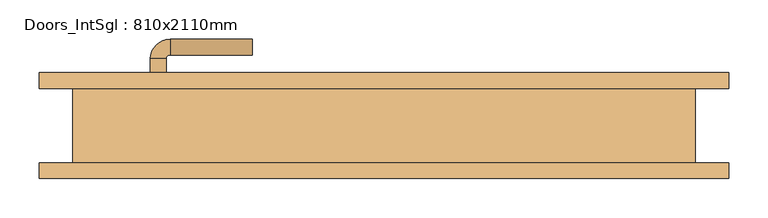
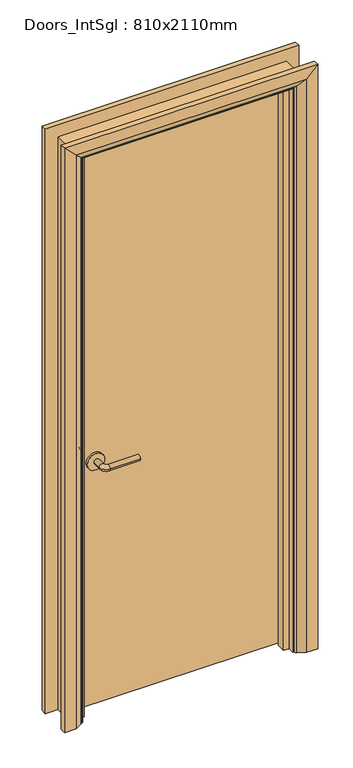
"""IFC4 building model written with IfcOpenShell, lengths in millimetres: door geometry, Doors_IntSgl : 810x2110mm."""

from ifc_helpers import new_model, si_unit, point, frame, frame_2d, origin, place, context, project, spatial, polyline, circle_curve, ellipse_curve, trimmed, segment, composite_curve, outline, extrude, faceted_brep, source, transform, mapped, element, save
from ifc_brep_helpers import plane_surface, cylinder_surface, revolved_surface, advanced_brep


def doors_intsgl_810x2110mm_acea5367(model_context):
    return source(origin(), model_context, "Body", "SolidModel", [
        advanced_brep(
        [(-298.0, 1.5, 900.0), (-278.0, 1.5, 900.0), (-278.0, -28.5, 900.0), (-298.0, -28.5, 900.0), (-273.0, -33.5, 900.0), (-273.0, -53.5, 900.0), (-168.0, -53.5, 900.0), (-168.0, -33.5, 900.0)],
        [
            (0, 1, circle_curve(frame((-288.0, 1.5, 900.0), z_axis=(0.0, 1.0, 0.0), x_axis=(1.0, 0.0, 0.0)), 10.0)),
            (1, 0, circle_curve(frame((-288.0, 1.5, 900.0), z_axis=(0.0, 1.0, 0.0), x_axis=(1.0, 0.0, 0.0)), 10.0)),
            (1, 2),
            (2, 3, circle_curve(frame((-288.0, -28.5, 900.0), z_axis=(0.0, 1.0, 0.0), x_axis=(1.0, 0.0, 0.0)), 10.0)),
            (3, 0),
            (3, 2, circle_curve(frame((-288.0, -28.5, 900.0), z_axis=(0.0, 1.0, 0.0), x_axis=(1.0, 0.0, 0.0)), 10.0)),
            (4, 5, circle_curve(frame((-273.0, -43.5, 900.0), z_axis=(-1.0, 0.0, 0.0), x_axis=(0.0, 1.0, 0.0)), 10.0)),
            (5, 3, circle_curve(frame((-273.0, -28.5, 900.0), z_axis=(0.0, 0.0, -1.0), x_axis=(-1.0, 0.0, 0.0)), 25.0)),
            (2, 4, circle_curve(frame((-273.0, -28.5, 900.0), z_axis=(0.0, 0.0, 1.0), x_axis=(-1.0, 0.0, 0.0)), 5.0)),
            (5, 4, circle_curve(frame((-273.0, -43.5, 900.0), z_axis=(-1.0, 0.0, 0.0), x_axis=(0.0, 1.0, 0.0)), 10.0)),
            (6, 7, circle_curve(frame((-168.0, -43.5, 900.0), z_axis=(1.0, 0.0, 0.0), x_axis=(0.0, 1.0, 0.0)), 10.0)),
            (7, 6, circle_curve(frame((-168.0, -43.5, 900.0), z_axis=(1.0, 0.0, 0.0), x_axis=(0.0, 1.0, 0.0)), 10.0)),
            (4, 7),
            (6, 5),
        ],
        [
            plane_surface(frame((-288.0, 1.5, 900.0), z_axis=(0.0, 1.0, 0.0), x_axis=(0.0, 0.0, 1.0))),
            cylinder_surface(frame((-288.0, 1.5, 900.0), z_axis=(0.0, 1.0, 0.0), x_axis=(1.0, 0.0, 0.0)), 10.0),
            revolved_surface(trimmed(ellipse_curve(frame((-288.0, -28.5, 900.0), z_axis=(0.0, -1.0, 0.0), x_axis=(1.0, 0.0, 0.0)), 10.0, 10.0), [point((-298.0, -28.5, 900.0))], [point((-278.0, -28.5, 900.0))], True, "CARTESIAN"), (-273.0, -28.5, 900.0), (0.0, 0.0, -1.0)),
            revolved_surface(trimmed(ellipse_curve(frame((-288.0, -28.5, 900.0), z_axis=(0.0, -1.0, 0.0), x_axis=(1.0, 0.0, 0.0)), 10.0, 10.0), [point((-278.0, -28.5, 900.0))], [point((-298.0, -28.5, 900.0))], True, "CARTESIAN"), (-273.0, -28.5, 900.0), (0.0, 0.0, -1.0)),
            plane_surface(frame((-168.0, -43.5, 900.0), z_axis=(1.0, 0.0, 0.0), x_axis=(0.0, 0.0, 1.0))),
            cylinder_surface(frame((-273.0, -43.5, 900.0), z_axis=(-1.0, 0.0, 0.0), x_axis=(0.0, 1.0, 0.0)), 10.0),
        ],
        [
            (0, [[1, 2]]),
            (1, [[3, 4, 5, -2]]),
            (1, [[-5, 6, -3, -1]]),
            (2, [[7, 8, -4, 9]]),
            (3, [[10, -9, -6, -8]]),
            (4, [[11, 12]]),
            (5, [[13, -11, 14, -7]]),
            (5, [[-14, -12, -13, -10]]),
        ],
    ),
        extrude(outline(composite_curve([segment(trimmed(circle_curve(frame_2d((900.0, -290.5)), 30.0), [point((900.0, -320.5))], [point((900.0, -260.5))], False, "CARTESIAN"), True, "CONTINUOUS"), segment(trimmed(circle_curve(frame_2d((900.0, -290.5)), 30.0), [point((900.0, -260.5))], [point((900.0, -320.5))], False, "CARTESIAN"), True, "CONTINUOUS")], self_intersect=False)), frame((0.0, 1.5, 0.0), z_axis=(0.0, 1.0, 0.0), x_axis=(0.0, 0.0, 1.0)), (0.0, 0.0, 1.0), 8.0),
        advanced_brep(
        [(-298.0, 55.5, 900.0), (-278.0, 55.5, 900.0), (-298.0, 85.5, 900.0), (-278.0, 85.5, 900.0), (-273.0, 90.5, 900.0), (-273.0, 110.5, 900.0), (-168.0, 110.5, 900.0), (-168.0, 90.5, 900.0)],
        [
            (0, 1, circle_curve(frame((-288.0, 55.5, 900.0), z_axis=(0.0, -1.0, 0.0), x_axis=(1.0, 0.0, 0.0)), 10.0)),
            (1, 0, circle_curve(frame((-288.0, 55.5, 900.0), z_axis=(0.0, -1.0, 0.0), x_axis=(1.0, 0.0, 0.0)), 10.0)),
            (0, 2),
            (2, 3, circle_curve(frame((-288.0, 85.5, 900.0), z_axis=(0.0, -1.0, 0.0), x_axis=(1.0, 0.0, 0.0)), 10.0)),
            (3, 1),
            (3, 2, circle_curve(frame((-288.0, 85.5, 900.0), z_axis=(0.0, -1.0, 0.0), x_axis=(1.0, 0.0, 0.0)), 10.0)),
            (4, 3, circle_curve(frame((-273.0, 85.5, 900.0), z_axis=(0.0, 0.0, 1.0), x_axis=(-1.0, 0.0, 0.0)), 5.0)),
            (2, 5, circle_curve(frame((-273.0, 85.5, 900.0), z_axis=(0.0, 0.0, -1.0), x_axis=(-1.0, 0.0, 0.0)), 25.0)),
            (5, 4, circle_curve(frame((-273.0, 100.5, 900.0), z_axis=(-1.0, 0.0, 0.0), x_axis=(0.0, -1.0, 0.0)), 10.0)),
            (4, 5, circle_curve(frame((-273.0, 100.5, 900.0), z_axis=(-1.0, 0.0, 0.0), x_axis=(0.0, -1.0, 0.0)), 10.0)),
            (6, 7, circle_curve(frame((-168.0, 100.5, 900.0), z_axis=(1.0, 0.0, 0.0), x_axis=(0.0, -1.0, 0.0)), 10.0)),
            (7, 6, circle_curve(frame((-168.0, 100.5, 900.0), z_axis=(1.0, 0.0, 0.0), x_axis=(0.0, -1.0, 0.0)), 10.0)),
            (5, 6),
            (7, 4),
        ],
        [
            plane_surface(frame((-288.0, 55.5, 900.0), z_axis=(0.0, -1.0, 0.0), x_axis=(0.0, 0.0, 1.0))),
            cylinder_surface(frame((-288.0, 55.5, 900.0), z_axis=(0.0, -1.0, 0.0), x_axis=(1.0, 0.0, 0.0)), 10.0),
            revolved_surface(trimmed(ellipse_curve(frame((-288.0, 85.5, 900.0), z_axis=(0.0, -1.0, 0.0), x_axis=(1.0, 0.0, 0.0)), 10.0, 10.0), [point((-298.0, 85.5, 900.0))], [point((-278.0, 85.5, 900.0))], True, "CARTESIAN"), (-273.0, 85.5, 900.0), (0.0, 0.0, -1.0)),
            revolved_surface(trimmed(ellipse_curve(frame((-288.0, 85.5, 900.0), z_axis=(0.0, -1.0, 0.0), x_axis=(1.0, 0.0, 0.0)), 10.0, 10.0), [point((-278.0, 85.5, 900.0))], [point((-298.0, 85.5, 900.0))], True, "CARTESIAN"), (-273.0, 85.5, 900.0), (0.0, 0.0, -1.0)),
            plane_surface(frame((-168.0, 100.5, 900.0), z_axis=(1.0, 0.0, 0.0), x_axis=(0.0, 0.0, 1.0))),
            cylinder_surface(frame((-273.0, 100.5, 900.0), z_axis=(-1.0, 0.0, 0.0), x_axis=(0.0, -1.0, 0.0)), 10.0),
        ],
        [
            (0, [[1, 2]]),
            (1, [[-1, 3, 4, 5]]),
            (1, [[-2, -5, 6, -3]]),
            (2, [[7, -4, 8, 9]]),
            (3, [[-8, -6, -7, 10]]),
            (4, [[11, 12]]),
            (5, [[-9, 13, -12, 14]]),
            (5, [[-10, -14, -11, -13]]),
        ],
    ),
        extrude(outline(composite_curve([segment(trimmed(circle_curve(frame_2d((900.0, -290.5)), 30.0), [point((900.0, -320.5))], [point((900.0, -260.5))], False, "CARTESIAN"), True, "CONTINUOUS"), segment(trimmed(circle_curve(frame_2d((900.0, -290.5)), 30.0), [point((900.0, -260.5))], [point((900.0, -320.5))], False, "CARTESIAN"), True, "CONTINUOUS")], self_intersect=False)), frame((0.0, 47.5, 0.0), z_axis=(0.0, 1.0, 0.0), x_axis=(0.0, 0.0, 1.0)), (0.0, 0.0, 1.0), 8.0),
        extrude(outline(polyline([(363.0, 9.5), (-363.0, 9.5), (-363.0, 47.5), (363.0, 47.5), (363.0, 9.5)])), frame((0.0, 0.0, 8.0), z_axis=(0.0, 0.0, 1.0), x_axis=(1.0, 0.0, 0.0)), (0.0, 0.0, 1.0), 2060.0),
        advanced_brep(
        [(440.0, 67.5, 0.0), (440.0, 47.5, 0.0), (370.0, 47.5, 0.0), (374.0, 53.5, 0.0), (400.0, 67.5, 0.0), (440.0, 67.5, 2145.0), (440.0, 47.5, 2145.0), (-440.0, 47.5, 2145.0), (-440.0, 47.5, 0.0), (-370.0, 47.5, 0.0), (-370.0, 47.5, 2075.0), (370.0, 47.5, 2075.0), (374.0, 53.5, 2079.0), (400.0, 67.5, 2105.0), (-400.0, 67.5, 2105.0), (-400.0, 67.5, 0.0), (-440.0, 67.5, 0.0), (-440.0, 67.5, 2145.0), (-374.0, 53.5, 2079.0), (-374.0, 53.5, 0.0)],
        [
            (0, 1),
            (1, 2),
            (2, 3, circle_curve(frame((378.0, 46.5, 0.0), z_axis=(0.0, 0.0, -1.0), x_axis=(1.0, 0.0, 0.0)), 8.0622577)),
            (3, 4),
            (4, 0),
            (0, 5),
            (5, 6),
            (6, 1),
            (6, 7),
            (7, 8),
            (8, 9),
            (9, 10),
            (10, 11),
            (11, 2),
            (11, 12, ellipse_curve(frame((378.0, 46.5, 2083.0), z_axis=(0.7071067811865475, 0.0, -0.7071067811865475), x_axis=(-0.7071067811865474, 0.0, -0.7071067811865476)), 11.4017543, 8.0622577)),
            (12, 3),
            (12, 13),
            (13, 4),
            (13, 14),
            (14, 15),
            (15, 16),
            (16, 17),
            (17, 5),
            (17, 7),
            (10, 18, ellipse_curve(frame((-378.0, 46.5, 2083.0), z_axis=(0.7071067811865475, 0.0, 0.7071067811865475), x_axis=(0.7071067811865476, 0.0, -0.7071067811865474)), 11.4017543, 8.0622577)),
            (18, 12),
            (18, 14),
            (15, 19),
            (19, 9, circle_curve(frame((-378.0, 46.5, 0.0), z_axis=(0.0, 0.0, -1.0), x_axis=(-1.0, 0.0, 0.0)), 8.0622577)),
            (8, 16),
            (19, 18),
        ],
        [
            plane_surface(frame((370.0, 47.5, 0.0), z_axis=(0.0, 0.0, -1.0), x_axis=(0.0, -1.0, 0.0))),
            plane_surface(frame((440.0, 67.5, 0.0), z_axis=(1.0, 0.0, 0.0), x_axis=(0.0, 0.0, 1.0))),
            plane_surface(frame((440.0, 47.5, 0.0), z_axis=(0.0, -1.0, 0.0), x_axis=(0.0, 0.0, 1.0))),
            cylinder_surface(frame((378.0, 46.5, 0.0), z_axis=(0.0, 0.0, -1.0), x_axis=(1.0, 0.0, 0.0)), 8.0622577),
            plane_surface(frame((374.0, 53.5, 0.0), z_axis=(-0.4740998230350126, 0.880471099922178, 0.0), x_axis=(0.0, 0.0, 1.0))),
            plane_surface(frame((400.0, 67.5, 0.0), z_axis=(0.0, 1.0, 0.0), x_axis=(0.0, 0.0, 1.0))),
            plane_surface(frame((440.0, 67.5, 2145.0), z_axis=(0.0, 0.0, 1.0), x_axis=(-1.0, 0.0, 0.0))),
            cylinder_surface(frame((370.0, 46.5, 2083.0), z_axis=(1.0, 0.0, 0.0), x_axis=(0.0, 0.0, 1.0)), 8.0622577),
            plane_surface(frame((374.0, 53.5, 2079.0), z_axis=(0.0, 0.8804710999221764, -0.4740998230350154), x_axis=(-1.0, 0.0, 0.0))),
            plane_surface(frame((-370.0, 47.5, 0.0), z_axis=(0.0, 0.0, -1.0), x_axis=(0.0, -1.0, 0.0))),
            plane_surface(frame((-440.0, 67.5, 2145.0), z_axis=(-1.0, 0.0, 0.0), x_axis=(0.0, 0.0, -1.0))),
            cylinder_surface(frame((-378.0, 46.5, 2075.0), z_axis=(0.0, 0.0, 1.0), x_axis=(-1.0, 0.0, 0.0)), 8.0622577),
            plane_surface(frame((-374.0, 53.5, 2079.0), z_axis=(0.47409982303501824, 0.8804710999221749, 0.0), x_axis=(0.0, 0.0, -1.0))),
        ],
        [
            (0, [[1, 2, 3, 4, 5]]),
            (1, [[-1, 6, 7, 8]]),
            (2, [[-2, -8, 9, 10, 11, 12, 13, 14]]),
            (3, [[-3, -14, 15, 16]]),
            (4, [[-4, -16, 17, 18]]),
            (5, [[-5, -18, 19, 20, 21, 22, 23, -6]]),
            (6, [[-7, -23, 24, -9]]),
            (7, [[-15, -13, 25, 26]]),
            (8, [[-17, -26, 27, -19]]),
            (9, [[-21, 28, 29, -11, 30]]),
            (10, [[-24, -22, -30, -10]]),
            (11, [[-25, -12, -29, 31]]),
            (12, [[-27, -31, -28, -20]]),
        ],
    ),
        extrude(outline(polyline([(0.0, -365.0), (0.0, -346.0), (2051.0, -346.0), (2051.0, 346.0), (0.0, 346.0), (0.0, 365.0), (2070.0, 365.0), (2070.0, -365.0), (0.0, -365.0)])), frame((0.0, -24.5, 0.0), z_axis=(0.0, 1.0, 0.0), x_axis=(0.0, 0.0, 1.0)), (0.0, 0.0, 1.0), 32.0),
        advanced_brep(
        [(-440.0, -67.5, 0.0), (-440.0, -47.5, 0.0), (-370.0, -47.5, 0.0), (-374.0, -53.5, 0.0), (-400.0, -67.5, 0.0), (-440.0, -67.5, 2145.0), (-440.0, -47.5, 2145.0), (-370.0, -47.5, 2075.0), (-374.0, -53.5, 2079.0), (-400.0, -67.5, 2105.0), (440.0, -67.5, 2145.0), (440.0, -47.5, 2145.0), (370.0, -47.5, 2075.0), (374.0, -53.5, 2079.0), (400.0, -67.5, 2105.0), (440.0, -67.5, 0.0), (400.0, -67.5, 0.0), (374.0, -53.5, 0.0), (370.0, -47.5, 0.0), (440.0, -47.5, 0.0)],
        [
            (0, 1),
            (1, 2),
            (2, 3, circle_curve(frame((-378.0, -46.5, 0.0), z_axis=(0.0, 0.0, -1.0), x_axis=(-1.0, 0.0, 0.0)), 8.0622577)),
            (3, 4),
            (4, 0),
            (0, 5),
            (5, 6),
            (6, 1),
            (6, 7),
            (7, 2),
            (7, 8, ellipse_curve(frame((-378.0, -46.5, 2083.0), z_axis=(-0.7071067811865475, 0.0, -0.7071067811865475), x_axis=(0.7071067811865474, 0.0, -0.7071067811865476)), 11.4017543, 8.0622577)),
            (8, 3),
            (8, 9),
            (9, 4),
            (9, 5),
            (5, 10),
            (10, 11),
            (11, 6),
            (11, 12),
            (12, 7),
            (12, 13, ellipse_curve(frame((378.0, -46.5, 2083.0), z_axis=(-0.7071067811865475, 0.0, 0.7071067811865475), x_axis=(-0.7071067811865476, 0.0, -0.7071067811865474)), 11.4017543, 8.0622577)),
            (13, 8),
            (13, 14),
            (14, 9),
            (14, 10),
            (15, 16),
            (16, 17),
            (17, 18, circle_curve(frame((378.0, -46.5, 0.0), z_axis=(0.0, 0.0, -1.0), x_axis=(1.0, 0.0, 0.0)), 8.0622577)),
            (18, 19),
            (19, 15),
            (10, 15),
            (19, 11),
            (18, 12),
            (17, 13),
            (16, 14),
        ],
        [
            plane_surface(frame((-370.0, -120.3010989, 0.0), z_axis=(0.0, 0.0, -1.0), x_axis=(1.0, 0.0, 0.0))),
            plane_surface(frame((-440.0, -67.5, 0.0), z_axis=(-1.0, 0.0, 0.0), x_axis=(0.0, 0.0, 1.0))),
            plane_surface(frame((-440.0, -47.5, 0.0), z_axis=(0.0, 1.0, 0.0), x_axis=(0.0, 0.0, 1.0))),
            cylinder_surface(frame((-378.0, -46.5, 0.0), z_axis=(0.0, 0.0, -1.0), x_axis=(-1.0, 0.0, 0.0)), 8.0622577),
            plane_surface(frame((-374.0, -53.5, 0.0), z_axis=(0.4740998230350183, -0.8804710999221749, 0.0), x_axis=(0.0, 0.0, 1.0))),
            plane_surface(frame((-400.0, -67.5, 0.0), z_axis=(0.0, -1.0, 0.0), x_axis=(0.0, 0.0, 1.0))),
            plane_surface(frame((-440.0, -67.5, 2145.0), z_axis=(0.0, 0.0, 1.0), x_axis=(1.0, 0.0, 0.0))),
            plane_surface(frame((-440.0, -47.5, 2145.0), z_axis=(0.0, 1.0, 0.0), x_axis=(1.0, 0.0, 0.0))),
            cylinder_surface(frame((-370.0, -46.5, 2083.0), z_axis=(-1.0, 0.0, 0.0), x_axis=(0.0, 0.0, 1.0)), 8.0622577),
            plane_surface(frame((-374.0, -53.5, 2079.0), z_axis=(0.0, -0.8804710999221749, -0.4740998230350183), x_axis=(1.0, 0.0, 0.0))),
            plane_surface(frame((-400.0, -67.5, 2105.0), z_axis=(0.0, -1.0, 0.0), x_axis=(1.0, 0.0, 0.0))),
            plane_surface(frame((370.0, -120.3010989, 0.0), z_axis=(0.0, 0.0, -1.0), x_axis=(-1.0, 0.0, 0.0))),
            plane_surface(frame((440.0, -67.5, 2145.0), z_axis=(1.0, 0.0, 0.0), x_axis=(0.0, 0.0, -1.0))),
            plane_surface(frame((440.0, -47.5, 2145.0), z_axis=(0.0, 1.0, 0.0), x_axis=(0.0, 0.0, -1.0))),
            cylinder_surface(frame((378.0, -46.5, 2075.0), z_axis=(0.0, 0.0, 1.0), x_axis=(1.0, 0.0, 0.0)), 8.0622577),
            plane_surface(frame((374.0, -53.5, 2079.0), z_axis=(-0.4740998230350183, -0.8804710999221749, 0.0), x_axis=(0.0, 0.0, -1.0))),
            plane_surface(frame((400.0, -67.5, 2105.0), z_axis=(0.0, -1.0, 0.0), x_axis=(0.0, 0.0, -1.0))),
        ],
        [
            (0, [[1, 2, 3, 4, 5]]),
            (1, [[-1, 6, 7, 8]]),
            (2, [[-2, -8, 9, 10]]),
            (3, [[-3, -10, 11, 12]]),
            (4, [[-4, -12, 13, 14]]),
            (5, [[-5, -14, 15, -6]]),
            (6, [[-7, 16, 17, 18]]),
            (7, [[-9, -18, 19, 20]]),
            (8, [[-11, -20, 21, 22]]),
            (9, [[-13, -22, 23, 24]]),
            (10, [[-15, -24, 25, -16]]),
            (11, [[26, 27, 28, 29, 30]]),
            (12, [[-17, 31, -30, 32]]),
            (13, [[-19, -32, -29, 33]]),
            (14, [[-21, -33, -28, 34]]),
            (15, [[-23, -34, -27, 35]]),
            (16, [[-25, -35, -26, -31]]),
        ],
    ),
        faceted_brep([(-365.0, 47.5, 0.0), (-365.0, -47.5, 0.0), (-397.0, -47.5, 0.0), (-397.0, 47.5, 0.0), (-365.0, 47.5, 2070.0), (-365.0, -47.5, 2070.0), (-397.0, -47.5, 2102.0), (-397.0, 47.5, 2102.0), (365.0, 47.5, 2070.0), (365.0, -47.5, 2070.0), (397.0, -47.5, 2102.0), (397.0, 47.5, 2102.0), (365.0, 47.5, 0.0), (397.0, 47.5, 0.0), (397.0, -47.5, 0.0), (365.0, -47.5, 0.0)], [[[0, 1, 2, 3]], [[1, 0, 4, 5]], [[2, 1, 5, 6]], [[3, 2, 6, 7]], [[0, 3, 7, 4]], [[5, 4, 8, 9]], [[6, 5, 9, 10]], [[7, 6, 10, 11]], [[4, 7, 11, 8]], [[12, 13, 14, 15]], [[9, 8, 12, 15]], [[10, 9, 15, 14]], [[11, 10, 14, 13]], [[8, 11, 13, 12]]]),
    ])


if __name__ == "__main__":
    model = new_model("IFC4")
    model_context = context("Model", 3, world=origin())
    ifc_project = project(units=[si_unit("LENGTHUNIT", "METRE", prefix="MILLI")], contexts=[model_context])
    site = spatial("IfcSite", under=ifc_project)
    building = spatial("IfcBuilding", under=site)
    placement = place(None, origin())
    doors_intsgl_810x2110mm_shape = doors_intsgl_810x2110mm_acea5367(model_context)
    element("IfcDoor", 1, ObjectType="Doors_IntSgl : 810x2110mm", at=placement, inside=building, context=model_context, shape_type="MappedRepresentation", body=[
        mapped(doors_intsgl_810x2110mm_shape, transform((0.0, 0.0, 0.0), x_axis=(1.0, 0.0, 0.0), y_axis=(0.0, 1.0, 0.0), z_axis=(0.0, 0.0, 1.0))),
    ])
    save(model, "model.ifc")

# Revit data of these elements
# Type "Doors_IntSgl : 810x2110mm"
#   Construction Type Id = "MDOOR"
#   Type Mark = "42"
#   Type Comments = "Internal Single"
#   Operation = "SingleSwingRight"
#   Manufacturer = "Revit"
#   Keynote = "L20"
#   Description = "Internal Single Door"
#   Analytic Construction = "Metal"
#   UnderCut = 8 mm
#   Tolerance = 2 mm
#   Thickness = 38 mm
#   Thermal Resistance (R) = 0.270117 (m²·K)/W
#   Structural Tolerance = 8 mm
#   StopDepth = 32 mm
#   Stop Thickness = 19 mm
#   Rough Width = 810 mm
#   Rough Height = 2110 mm
#   Height to Top Lock Rail = 1000 mm
#   Heat Transfer Coefficient (U) = 3.7021 W/(m²·K)
#   Handle Z Distance = 900 mm
#   Handle X Distance = 75 mm
#   Frame Thickness = 32 mm
#   Door Panel Width = 726 mm
#   Door Panel Thickness = 38 mm
#   Door Panel Offset = 0 mm
#   Height = 2110 mm
#   Width = 810 mm
#   Door Panel Height = 2060 mm
#   Architrave Setback = 5 mm
#   Vis - Ironmongery = yes
#   Material Ironmongery = Door - Handle
#   Material Frame = Door - Frame/Mullion (1)
#   Material Door = Door - Panel
#   Material Architrave = Door - Architrave
#   Visual Light Transmittance = 0
#   Solar Heat Gain Coefficient = 0
#   Function = (empty or 0)
#   Wall Closure = (empty or 0)
# Element 1 (IfcDoor, "Doors_IntSgl : 810x2110mm")
#   Materials on its faces: "Door - Architrave", "Door - Handle", "Door - Frame/Mullion (1)", "Door - Panel"
# Materials
#   "Door - Handle": class "Miscellaneous", colour RGB 0 0 0, transparency 0, Keynote = "P21"
#   "Door - Frame/Mullion (1)": class "Wood", colour RGB 212 179 113, transparency 0, Keynote = "L20", Cost = 0
#   "Door - Panel": class "Wood", colour RGB 210 159 95, transparency 0, Keynote = "L20"
#   "Door - Architrave": class "Wood", colour RGB 154 90 5, transparency 0, Keynote = "P20"
